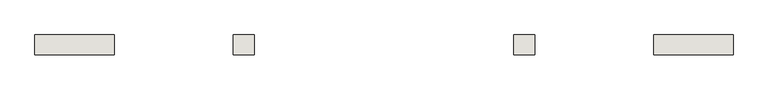
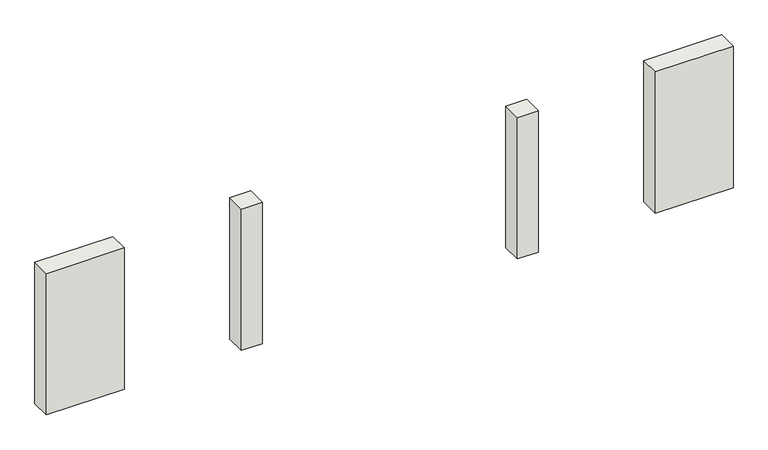
"""IFC4 building model written with IfcOpenShell, lengths in millimetres: wall geometry, 0_3d."""

from ifc_helpers import new_model, si_unit, origin, origin_with_axes, place, context, project, spatial, polyline, outline, extrude, source, transform, mapped, element, save


def wall_c1750b98(model_context):
    return source(origin(), model_context, "Body", "SweptSolid", [
        extrude(outline(polyline([(11740.0, 0.0), (11740.0, 380.0), (13240.0, 380.0), (13240.0, 0.0), (11740.0, 0.0)])), origin_with_axes(), (0.0, 0.0, 1.0), 2880.0),
        extrude(outline(polyline([(9080.0, 0.0), (9080.0, 380.0), (9480.0, 380.0), (9480.0, 0.0), (9080.0, 0.0)])), origin_with_axes(), (0.0, 0.0, 1.0), 2880.0),
        extrude(outline(polyline([(4160.0, 380.0), (4160.0, 0.0), (3760.0, 0.0), (3760.0, 380.0), (4160.0, 380.0)])), origin_with_axes(), (0.0, 0.0, 1.0), 2880.0),
        extrude(outline(polyline([(1500.0, 380.0), (1500.0, 0.0), (0.0, 0.0), (0.0, 380.0), (1500.0, 380.0)])), origin_with_axes(), (0.0, 0.0, 1.0), 2880.0),
    ])


if __name__ == "__main__":
    model = new_model("IFC4")
    model_context = context("Model", 3, world=origin())
    ifc_project = project(units=[si_unit("LENGTHUNIT", "METRE", prefix="MILLI")], contexts=[model_context])
    site = spatial("IfcSite", under=ifc_project)
    building = spatial("IfcBuilding", under=site)
    placement = place(None, origin())
    wall_shape = wall_c1750b98(model_context)
    element("IfcWall", 1, ObjectType="0_3d", at=placement, inside=building, context=model_context, shape_type="MappedRepresentation", body=[
        mapped(wall_shape, transform((0.0, 0.0, 0.0), x_axis=(1.0, 0.0, 0.0), y_axis=(0.0, 1.0, 0.0), z_axis=(0.0, 0.0, 1.0))),
    ])
    save(model, "model.ifc")

# Revit data of these elements
# Element 1 (IfcWall, "0_3d")
#   Materials on its faces: "holzschalung"
# Materials
#   "holzschalung": class "Unassigned", colour RGB 128 128 128, transparency 0
